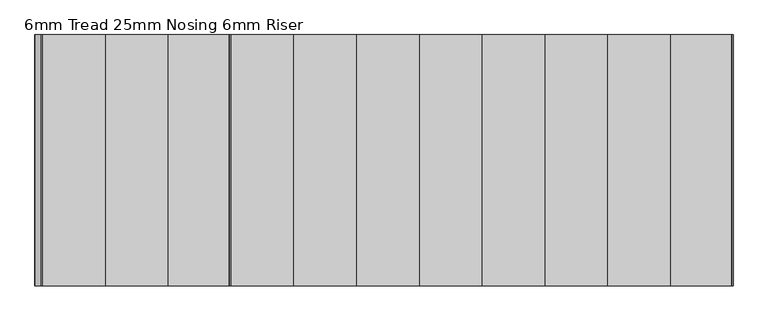
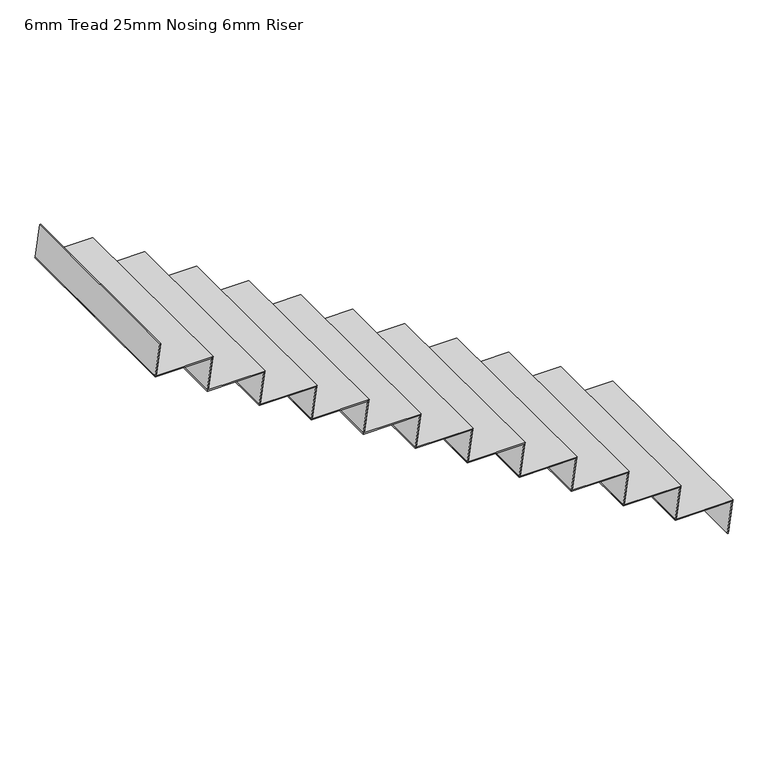
"""IFC4 building model written with IfcOpenShell, lengths in millimetres: stair flight geometry, 6mm Tread 25mm Nosing 6mm Riser."""

from ifc_helpers import new_model, si_unit, frame, origin, place, context, project, spatial, polyline, outline, extrude, source, transform, mapped, element, save


def stair_flight_6mm_tread_25mm_nosing_6mm_riser_93624e49(model_context):
    return source(origin(), model_context, "Body", "SweptSolid", [
        extrude(outline(polyline([(22294.1176471, 16350.0), (22294.1176471, 16043.9400908), (22288.1176471, 16043.0900908), (22288.1176471, 16349.15), (22294.1176471, 16350.0)])), frame((0.0, 12075.4345331, 0.0), z_axis=(0.0, 1.0, 0.0), x_axis=(0.0, 0.0, 1.0)), (0.0, 0.0, 1.0), 1100.0),
        extrude(outline(polyline([(22288.1176471, 16349.15), (22288.1176471, 16343.0900908), (22117.6470588, 16318.9400908), (22117.6470588, 16325.0), (22288.1176471, 16349.15)])), frame((0.0, 12075.4345331, 0.0), z_axis=(0.0, 1.0, 0.0), x_axis=(0.0, 0.0, 1.0)), (0.0, 0.0, 1.0), 1100.0),
        extrude(outline(polyline([(22464.5882353, 16074.15), (22464.5882353, 16068.0900908), (22294.1176471, 16043.9400908), (22294.1176471, 16050.0), (22464.5882353, 16074.15)])), frame((0.0, 12075.4345331, 0.0), z_axis=(0.0, 1.0, 0.0), x_axis=(0.0, 0.0, 1.0)), (0.0, 0.0, 1.0), 1100.0),
        extrude(outline(polyline([(22470.5882353, 16075.0), (22470.5882353, 15768.9400908), (22464.5882353, 15768.0900908), (22464.5882353, 16074.15), (22470.5882353, 16075.0)])), frame((0.0, 12075.4345331, 0.0), z_axis=(0.0, 1.0, 0.0), x_axis=(0.0, 0.0, 1.0)), (0.0, 0.0, 1.0), 1100.0),
        extrude(outline(polyline([(22641.0588235, 15799.15), (22641.0588235, 15793.0900908), (22470.5882353, 15768.9400908), (22470.5882353, 15775.0), (22641.0588235, 15799.15)])), frame((0.0, 12075.4345331, 0.0), z_axis=(0.0, 1.0, 0.0), x_axis=(0.0, 0.0, 1.0)), (0.0, 0.0, 1.0), 1100.0),
        extrude(outline(polyline([(22647.0588235, 15800.0), (22647.0588235, 15493.9400908), (22641.0588235, 15493.0900908), (22641.0588235, 15799.15), (22647.0588235, 15800.0)])), frame((0.0, 12075.4345331, 0.0), z_axis=(0.0, 1.0, 0.0), x_axis=(0.0, 0.0, 1.0)), (0.0, 0.0, 1.0), 1100.0),
        extrude(outline(polyline([(22817.5294118, 15524.15), (22817.5294118, 15518.0900908), (22647.0588235, 15493.9400908), (22647.0588235, 15500.0), (22817.5294118, 15524.15)])), frame((0.0, 12075.4345331, 0.0), z_axis=(0.0, 1.0, 0.0), x_axis=(0.0, 0.0, 1.0)), (0.0, 0.0, 1.0), 1100.0),
        extrude(outline(polyline([(22823.5294118, 15525.0), (22823.5294118, 15218.9400908), (22817.5294118, 15218.0900908), (22817.5294118, 15524.15), (22823.5294118, 15525.0)])), frame((0.0, 12075.4345331, 0.0), z_axis=(0.0, 1.0, 0.0), x_axis=(0.0, 0.0, 1.0)), (0.0, 0.0, 1.0), 1100.0),
        extrude(outline(polyline([(22994.0, 15249.15), (22994.0, 15243.0900908), (22823.5294118, 15218.9400908), (22823.5294118, 15225.0), (22994.0, 15249.15)])), frame((0.0, 12075.4345331, 0.0), z_axis=(0.0, 1.0, 0.0), x_axis=(0.0, 0.0, 1.0)), (0.0, 0.0, 1.0), 1100.0),
        extrude(outline(polyline([(23000.0, 15250.0), (23000.0, 14943.9400908), (22994.0, 14943.0900908), (22994.0, 15249.15), (23000.0, 15250.0)])), frame((0.0, 12075.4345331, 0.0), z_axis=(0.0, 1.0, 0.0), x_axis=(0.0, 0.0, 1.0)), (0.0, 0.0, 1.0), 1100.0),
        extrude(outline(polyline([(23170.4705882, 14974.15), (23170.4705882, 14968.0900908), (23000.0, 14943.9400908), (23000.0, 14950.0), (23170.4705882, 14974.15)])), frame((0.0, 12075.4345331, 0.0), z_axis=(0.0, 1.0, 0.0), x_axis=(0.0, 0.0, 1.0)), (0.0, 0.0, 1.0), 1100.0),
        extrude(outline(polyline([(23176.4705882, 14975.0), (23176.4705882, 14668.9400908), (23170.4705882, 14668.0900908), (23170.4705882, 14974.15), (23176.4705882, 14975.0)])), frame((0.0, 12075.4345331, 0.0), z_axis=(0.0, 1.0, 0.0), x_axis=(0.0, 0.0, 1.0)), (0.0, 0.0, 1.0), 1100.0),
        extrude(outline(polyline([(23346.9411765, 14699.15), (23346.9411765, 14693.0900908), (23176.4705882, 14668.9400908), (23176.4705882, 14675.0), (23346.9411765, 14699.15)])), frame((0.0, 12075.4345331, 0.0), z_axis=(0.0, 1.0, 0.0), x_axis=(0.0, 0.0, 1.0)), (0.0, 0.0, 1.0), 1100.0),
        extrude(outline(polyline([(23352.9411765, 14700.0), (23352.9411765, 14393.9400908), (23346.9411765, 14393.0900908), (23346.9411765, 14699.15), (23352.9411765, 14700.0)])), frame((0.0, 12075.4345331, 0.0), z_axis=(0.0, 1.0, 0.0), x_axis=(0.0, 0.0, 1.0)), (0.0, 0.0, 1.0), 1100.0),
        extrude(outline(polyline([(23523.4117647, 14424.15), (23523.4117647, 14418.0900908), (23352.9411765, 14393.9400908), (23352.9411765, 14400.0), (23523.4117647, 14424.15)])), frame((0.0, 12075.4345331, 0.0), z_axis=(0.0, 1.0, 0.0), x_axis=(0.0, 0.0, 1.0)), (0.0, 0.0, 1.0), 1100.0),
        extrude(outline(polyline([(23529.4117647, 14425.0), (23529.4117647, 14118.9400908), (23523.4117647, 14118.0900908), (23523.4117647, 14424.15), (23529.4117647, 14425.0)])), frame((0.0, 12075.4345331, 0.0), z_axis=(0.0, 1.0, 0.0), x_axis=(0.0, 0.0, 1.0)), (0.0, 0.0, 1.0), 1100.0),
        extrude(outline(polyline([(23699.8823529, 14149.15), (23699.8823529, 14143.0900908), (23529.4117647, 14118.9400908), (23529.4117647, 14125.0), (23699.8823529, 14149.15)])), frame((0.0, 12075.4345331, 0.0), z_axis=(0.0, 1.0, 0.0), x_axis=(0.0, 0.0, 1.0)), (0.0, 0.0, 1.0), 1100.0),
        extrude(outline(polyline([(23705.8823529, 14150.0), (23705.8823529, 13843.9400908), (23699.8823529, 13843.0900908), (23699.8823529, 14149.15), (23705.8823529, 14150.0)])), frame((0.0, 12075.4345331, 0.0), z_axis=(0.0, 1.0, 0.0), x_axis=(0.0, 0.0, 1.0)), (0.0, 0.0, 1.0), 1100.0),
        extrude(outline(polyline([(23876.3529412, 13874.15), (23876.3529412, 13868.0900908), (23705.8823529, 13843.9400908), (23705.8823529, 13850.0), (23876.3529412, 13874.15)])), frame((0.0, 12075.4345331, 0.0), z_axis=(0.0, 1.0, 0.0), x_axis=(0.0, 0.0, 1.0)), (0.0, 0.0, 1.0), 1100.0),
        extrude(outline(polyline([(23882.3529412, 13875.0), (23882.3529412, 13568.9400908), (23876.3529412, 13568.0900908), (23876.3529412, 13874.15), (23882.3529412, 13875.0)])), frame((0.0, 12075.4345331, 0.0), z_axis=(0.0, 1.0, 0.0), x_axis=(0.0, 0.0, 1.0)), (0.0, 0.0, 1.0), 1100.0),
        extrude(outline(polyline([(24052.8235294, 13599.15), (24052.8235294, 13593.0900908), (23882.3529412, 13568.9400908), (23882.3529412, 13575.0), (24052.8235294, 13599.15)])), frame((0.0, 12075.4345331, 0.0), z_axis=(0.0, 1.0, 0.0), x_axis=(0.0, 0.0, 1.0)), (0.0, 0.0, 1.0), 1100.0),
        extrude(outline(polyline([(24229.2941176, 13324.15), (24229.2941176, 13318.0900908), (24058.8235294, 13293.9400908), (24058.8235294, 13300.0), (24229.2941176, 13324.15)])), frame((0.0, 12075.4345331, 0.0), z_axis=(0.0, 1.0, 0.0), x_axis=(0.0, 0.0, 1.0)), (0.0, 0.0, 1.0), 1100.0),
        extrude(outline(polyline([(24058.8235294, 13600.0), (24058.8235294, 13293.9400908), (24052.8235294, 13293.0900908), (24052.8235294, 13599.15), (24058.8235294, 13600.0)])), frame((0.0, 12075.4345331, 0.0), z_axis=(0.0, 1.0, 0.0), x_axis=(0.0, 0.0, 1.0)), (0.0, 0.0, 1.0), 1100.0),
    ])


if __name__ == "__main__":
    model = new_model("IFC4")
    model_context = context("Model", 3, world=origin())
    ifc_project = project(units=[si_unit("LENGTHUNIT", "METRE", prefix="MILLI")], contexts=[model_context])
    site = spatial("IfcSite", under=ifc_project)
    building = spatial("IfcBuilding", under=site)
    placement = place(None, origin())
    stair_flight_6mm_tread_25mm_nosing_6mm_riser_shape = stair_flight_6mm_tread_25mm_nosing_6mm_riser_93624e49(model_context)
    element("IfcStairFlight", 1, ObjectType="6mm Tread 25mm Nosing 6mm Riser", at=placement, inside=building, context=model_context, shape_type="MappedRepresentation", body=[
        mapped(stair_flight_6mm_tread_25mm_nosing_6mm_riser_shape, transform((0.0, 0.0, 0.0), x_axis=(1.0, 0.0, 0.0), y_axis=(0.0, 1.0, 0.0), z_axis=(0.0, 0.0, 1.0))),
    ])
    save(model, "model.ifc")

# Revit data of these elements
# Element 1 (IfcStairFlight, "6mm Tread 25mm Nosing 6mm Riser")
#   Materials on its faces: "Steel, Paint Finish, Dark Gray"
# Materials
#   "Steel, Paint Finish, Dark Gray": class "Metal", colour RGB 89 89 89, transparency 0, Description = "Steel, paint finish, dark gray, glossy", Cost = 0
